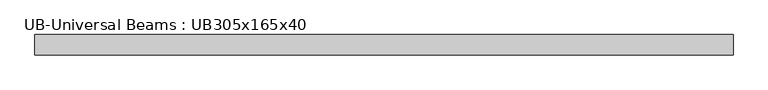
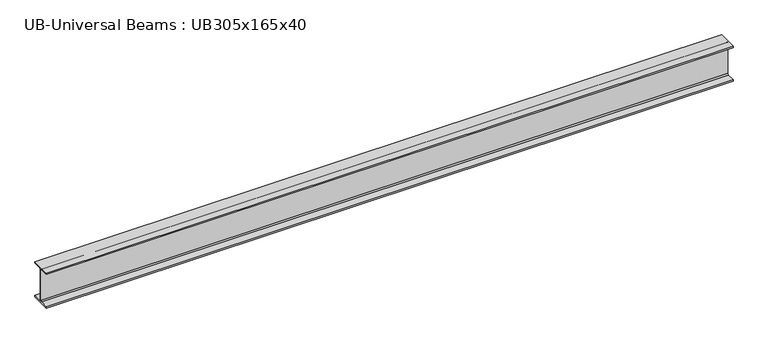
"""IFC4 building model written with IfcOpenShell, lengths in millimetres: beam geometry, UB-Universal Beams : UB305x165x40."""

from ifc_helpers import new_model, si_unit, point, frame, frame_2d, origin, place, context, project, spatial, polyline, circle_curve, trimmed, segment, composite_curve, outline, extrude, source, transform, mapped, element, save


def ub_universal_beams_ub305x165x40_4fbda082(model_context):
    return source(origin(), model_context, "Body", "SweptSolid", [
        extrude(outline(composite_curve([segment(polyline([(82.5, -141.5), (82.5, -151.7), (-82.5, -151.7), (-82.5, -141.5), (-11.9, -141.5)]), True, "CONTINUOUS"), segment(trimmed(circle_curve(frame_2d((-11.9, -132.6)), 8.9), [point((-11.9, -141.5))], [point((-3.0, -132.6))], True, "CARTESIAN"), True, "CONTINUOUS"), segment(polyline([(-3.0, -132.6), (-3.0, 132.6)]), True, "CONTINUOUS"), segment(trimmed(circle_curve(frame_2d((-11.9, 132.6)), 8.9), [point((-3.0, 132.6))], [point((-11.9, 141.5))], True, "CARTESIAN"), True, "CONTINUOUS"), segment(polyline([(-11.9, 141.5), (-82.5, 141.5), (-82.5, 151.7), (82.5, 151.7), (82.5, 141.5), (11.9, 141.5)]), True, "CONTINUOUS"), segment(trimmed(circle_curve(frame_2d((11.9, 132.6)), 8.9), [point((11.9, 141.5))], [point((3.0, 132.6))], True, "CARTESIAN"), True, "CONTINUOUS"), segment(polyline([(3.0, 132.6), (3.0, -132.6)]), True, "CONTINUOUS"), segment(trimmed(circle_curve(frame_2d((11.9, -132.6)), 8.9), [point((3.0, -132.6))], [point((11.9, -141.5))], True, "CARTESIAN"), True, "CONTINUOUS"), segment(polyline([(11.9, -141.5), (82.5, -141.5)]), True, "CONTINUOUS")], self_intersect=False)), frame((-2834.6, 0.0, 0.0), z_axis=(1.0, 0.0, 0.0), x_axis=(0.0, 1.0, 0.0)), (0.0, 0.0, 1.0), 5669.2),
    ])


if __name__ == "__main__":
    model = new_model("IFC4")
    model_context = context("Model", 3, world=origin())
    ifc_project = project(units=[si_unit("LENGTHUNIT", "METRE", prefix="MILLI")], contexts=[model_context])
    site = spatial("IfcSite", under=ifc_project)
    building = spatial("IfcBuilding", under=site)
    placement = place(None, origin())
    ub_universal_beams_ub305x165x40_shape = ub_universal_beams_ub305x165x40_4fbda082(model_context)
    element("IfcBeam", 1, ObjectType="UB-Universal Beams : UB305x165x40", at=placement, inside=building, context=model_context, shape_type="MappedRepresentation", body=[
        mapped(ub_universal_beams_ub305x165x40_shape, transform((0.0, 0.0, 0.0), x_axis=(1.0, 0.0, 0.0), y_axis=(0.0, 1.0, 0.0), z_axis=(0.0, 0.0, 1.0))),
    ])
    save(model, "model.ifc")

# Revit data of these elements
# Type "UB-Universal Beams : UB305x165x40"
#   Section Name Key = "UB305X165X40"
#   Width = 16.5 cm
#   Web Thickness = 0.6 cm
#   Web Fillet = 0.89 cm
#   Warping Constant = 164000.0 cm⁶
#   Torsional Moment of Inertia = 14.70 cm⁴
#   Section Area = 51.3 cm²
#   Plastic Modulus weak axis = 142.0 cm³
#   Plastic Modulus strong axis = 623.0 cm³
#   Nominal Weight = 40.2999 kgf/m
#   Moment of Inertia weak axis = 764.00 cm⁴
#   Moment of Inertia strong axis = 8503.00 cm⁴
#   Height = 30.34 cm
#   Flange Thickness = 1.02 cm
#   Elastic Modulus weak axis = 92.6 cm³
#   Elastic Modulus strong axis = 560.0 cm³
#   Centroid Vertical = 15.17 cm
#   Centroid Horizontal = 8.25 cm
#   Bolt Spacing = 9.0 cm
#   Length [instance default] = 1500 mm
#   Structural Material [instance default] = Metal - Steel 43-275
#   Type Comments = ""
#   Assembly Code = ""
# Element 1 (IfcBeam, "UB-Universal Beams : UB305x165x40")
#   Materials on its faces: "Metal - Steel 43-275"
# Materials
#   "Metal - Steel 43-275": class "Metal", colour RGB 247 247 247, transparency 0, Cost = 0
